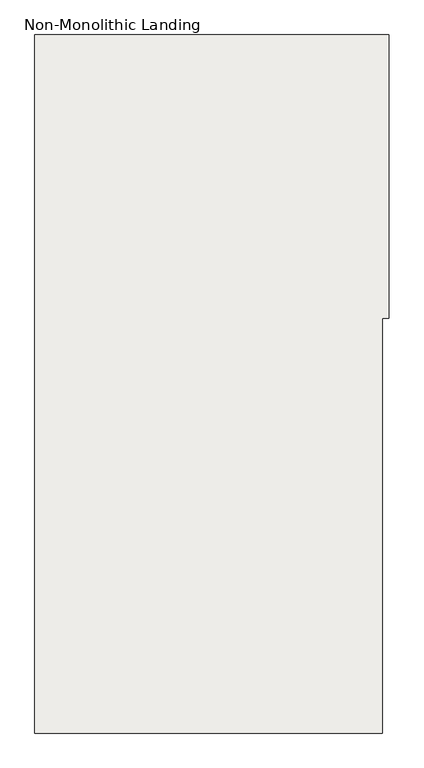
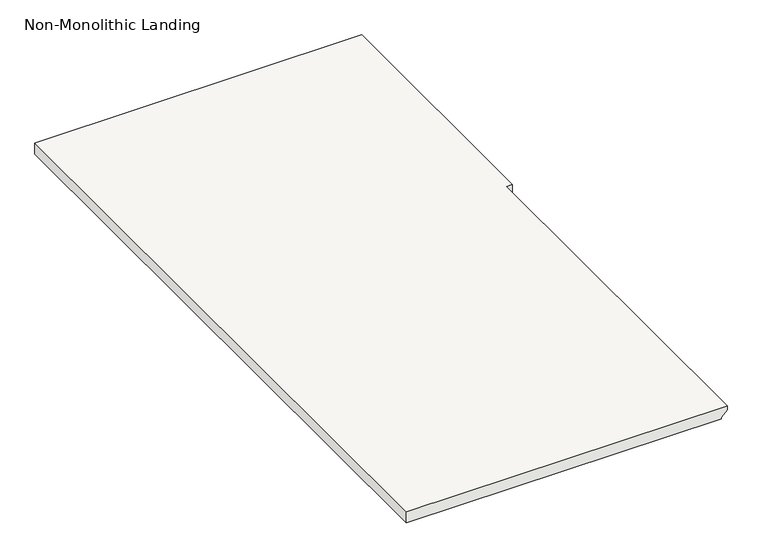
"""IFC4 building model written with IfcOpenShell, lengths in millimetres: slab geometry, Non-Monolithic Landing."""

import ifcopenshell
import ifcopenshell.guid

model = None  # the IFC model being written
_history = None  # IfcOwnerHistory: only IFC2X3 demands one
_inside = {}  # id of a spatial element -> (the spatial element, [elements in it])
_under = {}  # id of a project, library or spatial element -> (it, [spatial elements below it])
_declared = {}  # id of a project -> (the project, [libraries it declares])
_typed = {}  # id of a type object -> (the type object, [elements of that type])
_made_of = {}  # id of a material, layer set ... -> (it, [elements and type objects made of it])


def new_model(schema):
    """Start an empty IFC model of exactly this schema.

    Asked for "IFC4X3", IfcOpenShell would pick the latest addendum, in which some entities
    have other attributes; the version numbers below select the first issue.
    IFC2X3 requires an IfcOwnerHistory on every rooted entity: one is made here for all.
    """
    global model, _history
    if schema == "IFC4X3":
        model = ifcopenshell.file(schema_version=(4, 3, 0, 0))
    else:
        model = ifcopenshell.file(schema=schema)
    _inside.clear()
    _under.clear()
    _declared.clear()
    _typed.clear()
    _made_of.clear()
    _history = None
    if model.schema == "IFC2X3":
        org = make("IfcOrganization", Name="unknown")
        user = make(
            "IfcPersonAndOrganization",
            ThePerson=make("IfcPerson", FamilyName="unknown"),
            TheOrganization=org,
        )
        app = make(
            "IfcApplication",
            ApplicationDeveloper=org,
            Version="unknown",
            ApplicationFullName="unknown",
            ApplicationIdentifier="unknown",
        )
        _history = make(
            "IfcOwnerHistory",
            OwningUser=user,
            OwningApplication=app,
            ChangeAction="ADDED",
            CreationDate=0,
        )
    return model


def make(cls, **values):
    """One entity of the class cls with the attributes given. An attribute that is None is left unset."""
    return model.create_entity(
        cls, **{name: value for name, value in values.items() if value is not None}
    )


def rooted(cls, **values):
    """An entity with a GlobalId (a new one), such as an element, a storey or a relation."""
    return make(cls, GlobalId=ifcopenshell.guid.new(), OwnerHistory=_history, **values)


def si_unit(unit_type, name, prefix=None):
    """IfcSIUnit, for example si_unit("LENGTHUNIT", "METRE", prefix="MILLI")."""
    return make("IfcSIUnit", UnitType=unit_type, Prefix=prefix, Name=name)


def assignment(units):
    """IfcUnitAssignment: the units of a project."""
    return None if units is None else make("IfcUnitAssignment", Units=units)


def point(xyz):
    """IfcCartesianPoint."""
    return None if xyz is None else make("IfcCartesianPoint", Coordinates=xyz)


def direction(xyz):
    """IfcDirection."""
    return None if xyz is None else make("IfcDirection", DirectionRatios=xyz)


def frame(location, z_axis=None, x_axis=None):
    """IfcAxis2Placement3D, a coordinate frame: its origin and axes. An axis left out is left unset."""
    return make(
        "IfcAxis2Placement3D",
        Location=point(location),
        Axis=direction(z_axis),
        RefDirection=direction(x_axis),
    )


def origin():
    """The frame at (0, 0, 0) with its axes left unset."""
    return frame((0.0, 0.0, 0.0))


def place(relative_to, where):
    """IfcLocalPlacement: puts the frame where relative to a parent placement (None: the world)."""
    return make(
        "IfcLocalPlacement", PlacementRelTo=relative_to, RelativePlacement=where
    )


def context(
    kind, dimensions, precision=None, world=None, true_north=None, identifier=None
):
    """IfcGeometricRepresentationContext, for example the 3D "Model" context."""
    return make(
        "IfcGeometricRepresentationContext",
        ContextIdentifier=identifier,
        ContextType=kind,
        CoordinateSpaceDimension=dimensions,
        Precision=precision,
        WorldCoordinateSystem=world,
        TrueNorth=true_north,
    )


def project(units=None, contexts=None):
    """IfcProject with its units and contexts."""
    return rooted(
        "IfcProject",
        Name="project",
        RepresentationContexts=contexts,
        UnitsInContext=assignment(units),
    )


def spatial(cls, under=None, at=None, **own):
    """A site, building, storey or space (cls), placed at a placement, below another one or the project."""
    s = rooted(cls, ObjectPlacement=at, **own)
    if under is not None:
        _under.setdefault(under.id(), (under, []))[1].append(s)
    return s


def faces_of(points, faces, orient=None, outer=None):
    """IfcFace entities. A face is a list of loops; a loop is a list of indices into points, from 0.

    orient and outer hold one flag for each loop. By default every Orientation is true, the
    first loop of a face is its IfcFaceOuterBound and the others are IfcFaceBound.
    """
    made = []
    for i, loops in enumerate(faces):
        bounds = []
        for j, loop in enumerate(loops):
            is_outer = j == 0 if outer is None else outer[i][j]
            bounds.append(
                make(
                    "IfcFaceOuterBound" if is_outer else "IfcFaceBound",
                    Bound=make("IfcPolyLoop", Polygon=[points[k] for k in loop]),
                    Orientation=True if orient is None else orient[i][j],
                )
            )
        made.append(make("IfcFace", Bounds=bounds))
    return made


def faceted_brep(points, faces, orient=None, outer=None, voids=None):
    """IfcFacetedBrep: a solid bounded by flat faces; with voids (closed shells), ...WithVoids."""
    shared = [point(p) for p in points]
    hull = make("IfcClosedShell", CfsFaces=faces_of(shared, faces, orient, outer))
    if voids is None:
        return make("IfcFacetedBrep", Outer=hull)
    return make(
        "IfcFacetedBrepWithVoids",
        Outer=hull,
        Voids=[
            make(cls, CfsFaces=faces_of(shared, fs, o, b)) for cls, fs, o, b in voids
        ],
    )


def shape(context_of_items, identifier, shape_type, items):
    """IfcShapeRepresentation: the items that make up one representation, for example the "Body"."""
    return make(
        "IfcShapeRepresentation",
        ContextOfItems=context_of_items,
        RepresentationIdentifier=identifier,
        RepresentationType=shape_type,
        Items=items,
    )


def source(mapping_origin, context_of_items, identifier, shape_type, items):
    """IfcRepresentationMap: a shape defined once, which mapped items show again and again."""
    return make(
        "IfcRepresentationMap",
        MappingOrigin=mapping_origin,
        MappedRepresentation=shape(context_of_items, identifier, shape_type, items),
    )


def transform(
    local_origin,
    x_axis=None,
    y_axis=None,
    z_axis=None,
    scale=None,
    scale2=None,
    scale3=None,
    uniform=True,
):
    """IfcCartesianTransformationOperator3D, or its non-uniform kind. x_axis, y_axis, z_axis: its Axis1, 2, 3."""
    if uniform:
        return make(
            "IfcCartesianTransformationOperator3D",
            Axis1=direction(x_axis),
            Axis2=direction(y_axis),
            LocalOrigin=point(local_origin),
            Scale=scale,
            Axis3=direction(z_axis),
        )
    return make(
        "IfcCartesianTransformationOperator3DnonUniform",
        Axis1=direction(x_axis),
        Axis2=direction(y_axis),
        LocalOrigin=point(local_origin),
        Scale=scale,
        Axis3=direction(z_axis),
        Scale2=scale2,
        Scale3=scale3,
    )


def mapped(mapping_source, mapping_target):
    """IfcMappedItem: shows the shape of a source again, moved by a transform."""
    return make(
        "IfcMappedItem", MappingSource=mapping_source, MappingTarget=mapping_target
    )


def made_of(thing, what):
    """Note that an element or type object is made of a material, layer set ...; save() writes the relation."""
    if what is not None:
        _made_of.setdefault(what.id(), (what, []))[1].append(thing)
    return thing


def element(
    cls,
    number,
    at=None,
    inside=None,
    cuts=None,
    type_object=None,
    material=None,
    context=None,
    identifier="Body",
    shape_type=None,
    held_by="IfcProductDefinitionShape",
    body=None,
    shapes=None,
    **own,
):
    """One element of the class cls, such as IfcWall. Its Tag is "e" and its number.

    at: its placement. inside: the storey or other place that contains it. cuts: it is an
    opening in that element (IfcRelVoidsElement). A single representation is given by context,
    identifier, shape_type and body (its items); several are given by shapes. held_by: the class
    of the entity that holds the representations. save() writes the other relations.
    """
    e = rooted(cls, Tag="e%d" % number, ObjectPlacement=at, **own)
    if body is not None:
        shapes = [shape(context, identifier, shape_type, body)]
    if shapes is not None:
        e.Representation = make(held_by, Representations=shapes)
    if inside is not None:
        _inside.setdefault(inside.id(), (inside, []))[1].append(e)
    if cuts is not None:
        rooted(
            "IfcRelVoidsElement", RelatingBuildingElement=cuts, RelatedOpeningElement=e
        )
    if type_object is not None:
        _typed.setdefault(type_object.id(), (type_object, []))[1].append(e)
    return made_of(e, material)


def aggregate(whole, parts):
    """IfcRelAggregates: a whole, such as a stair, and the parts it consists of."""
    return rooted("IfcRelAggregates", RelatingObject=whole, RelatedObjects=parts)


def save(model, path):
    """Write the relations noted so far, then the file.

    IfcRelAggregates (storeys below a building ...), IfcRelContainedInSpatialStructure (elements
    in a storey), IfcRelDefinesByType, IfcRelAssociatesMaterial and IfcRelDeclares: one each for
    every whole, place, type object, material and project.
    """
    for whole, parts in _under.values():
        aggregate(whole, parts)
    for where, things in _inside.values():
        rooted(
            "IfcRelContainedInSpatialStructure",
            RelatedElements=things,
            RelatingStructure=where,
        )
    for kind, things in _typed.values():
        rooted("IfcRelDefinesByType", RelatedObjects=things, RelatingType=kind)
    for what, things in _made_of.values():
        rooted("IfcRelAssociatesMaterial", RelatedObjects=things, RelatingMaterial=what)
    for by, libraries in _declared.values():
        rooted("IfcRelDeclares", RelatingContext=by, RelatedDefinitions=libraries)
    model.write(path)


def non_monolithic_landing_cc7d3835(model_context):
    return source(origin(), model_context, "Body", "Brep", [
        faceted_brep([(-3502.6122732, 6497.5015304, 5554.4357143), (-3528.0122732, 6497.5015304, 5529.0357143), (-3528.0122732, 7615.1015304, 5529.0357143), (-3502.6122732, 7615.1015304, 5554.4357143), (-3502.6122732, 8132.6265304, 5573.4857143), (-3477.2122732, 8132.6265304, 5573.4857143), (-3477.2122732, 9250.2265304, 5573.4857143), (-3502.6122732, 9250.2265304, 5573.4857143), (-4874.2122732, 9250.2265304, 5573.4857143), (-4874.2122732, 6497.5015304, 5573.4857143), (-3502.6122732, 6497.5015304, 5573.4857143), (-3528.0122732, 7615.1015304, 5522.6857143), (-3528.0122732, 6497.5015304, 5522.6857143), (-4874.2122732, 6497.5015304, 5522.6857143), (-4874.2122732, 9250.2265304, 5522.6857143), (-3502.6122732, 9250.2265304, 5522.6857143), (-3477.2122732, 9250.2265304, 5522.6857143), (-3477.2122732, 8132.6265304, 5522.6857143), (-3502.6122732, 8132.6265304, 5522.6857143), (-3502.6122732, 7615.1015304, 5522.6857143)], [[[0, 1, 2, 3]], [[4, 5, 6, 7, 8, 9, 10]], [[11, 12, 13, 14, 15, 16, 17, 18, 19]], [[12, 11, 2, 1]], [[11, 19, 3, 2]], [[4, 10, 0, 3, 19, 18]], [[5, 4, 18, 17]], [[6, 5, 17, 16]], [[7, 6, 16, 15]], [[8, 7, 15, 14]], [[9, 8, 14, 13]], [[10, 9, 13, 12, 1, 0]]]),
    ])


if __name__ == "__main__":
    model = new_model("IFC4")
    model_context = context("Model", 3, world=origin())
    ifc_project = project(units=[si_unit("LENGTHUNIT", "METRE", prefix="MILLI")], contexts=[model_context])
    site = spatial("IfcSite", under=ifc_project)
    building = spatial("IfcBuilding", under=site)
    placement = place(None, origin())
    non_monolithic_landing_shape = non_monolithic_landing_cc7d3835(model_context)
    element("IfcSlab", 1, ObjectType="Non-Monolithic Landing", at=placement, inside=building, context=model_context, shape_type="MappedRepresentation", body=[
        mapped(non_monolithic_landing_shape, transform((0.0, 0.0, 0.0), x_axis=(1.0, 0.0, 0.0), y_axis=(0.0, 1.0, 0.0), z_axis=(0.0, 0.0, 1.0))),
    ])
    save(model, "model.ifc")

# Revit data of these elements
# Project information
#   Organization Name = "G3B Press"
#   Organization Description = "Paul F. Aubin Cosulting Services, Inc."
#   Building Name = "Revit Essentials for Architecture"
#   Author = "Paul F. Aubin"
#   Author Website = "https://www.paulaubin.com"
#   Copyright = "Copyright © 2020 Paul F Aubin, all rights reserved"
#   Design Option = "Main Model"
#   Project Issue Date = "8/1/2020"
#   Project Status = "Design Development"
#   Client Name = "Developing the Exterior Skin"
#   Project Address = "123 State ST\nSuite 301\nChicago, IL 60606"
#   Project Name = "10 Commercial"
#   Project Number = "2020.04A"
